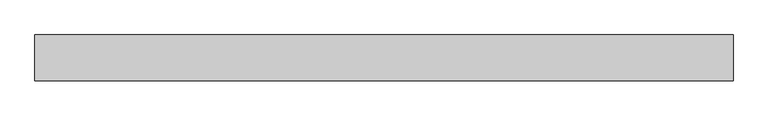
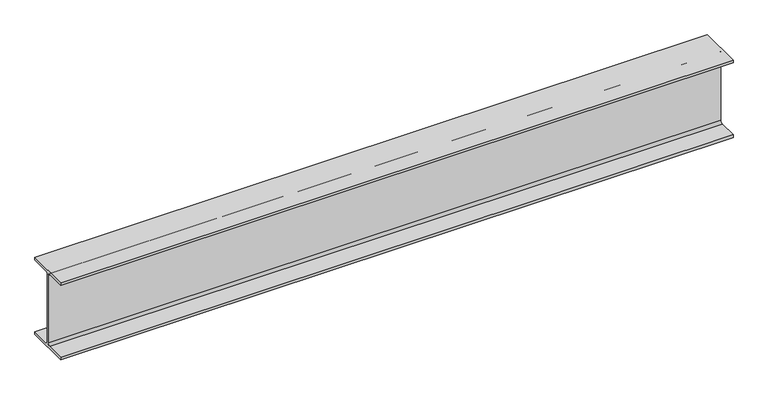
"""IFC4 building model written with IfcOpenShell, lengths in millimetres: beam geometry, Old_Steel Beam_H-KSD3502 : H_SB_ASB_H-200×200x8x12."""

from ifc_helpers import new_model, si_unit, point, frame, frame_2d, origin, place, context, project, spatial, polyline, circle_curve, trimmed, segment, composite_curve, outline, extrude, source, transform, mapped, element, save


def beam_1490ead7(model_context):
    return source(origin(), model_context, "Body", "SweptSolid", [
        extrude(outline(composite_curve([segment(polyline([(82.5, -141.5), (82.5, -151.7), (-82.5, -151.7), (-82.5, -141.5), (-11.9, -141.5)]), True, "CONTINUOUS"), segment(trimmed(circle_curve(frame_2d((-11.9, -132.6)), 8.9), [point((-11.9, -141.5))], [point((-3.0, -132.6))], True, "CARTESIAN"), True, "CONTINUOUS"), segment(polyline([(-3.0, -132.6), (-3.0, 132.6)]), True, "CONTINUOUS"), segment(trimmed(circle_curve(frame_2d((-11.9, 132.6)), 8.9), [point((-3.0, 132.6))], [point((-11.9, 141.5))], True, "CARTESIAN"), True, "CONTINUOUS"), segment(polyline([(-11.9, 141.5), (-82.5, 141.5), (-82.5, 151.7), (82.5, 151.7), (82.5, 141.5), (11.9, 141.5)]), True, "CONTINUOUS"), segment(trimmed(circle_curve(frame_2d((11.9, 132.6)), 8.9), [point((11.9, 141.5))], [point((3.0, 132.6))], True, "CARTESIAN"), True, "CONTINUOUS"), segment(polyline([(3.0, 132.6), (3.0, -132.6)]), True, "CONTINUOUS"), segment(trimmed(circle_curve(frame_2d((11.9, -132.6)), 8.9), [point((3.0, -132.6))], [point((11.9, -141.5))], True, "CARTESIAN"), True, "CONTINUOUS"), segment(polyline([(11.9, -141.5), (82.5, -141.5)]), True, "CONTINUOUS")], self_intersect=False)), frame((-1276.0000495, 0.0, 0.0), z_axis=(1.0, 0.0, 0.0), x_axis=(0.0, 1.0, 0.0)), (0.0, 0.0, 1.0), 2501.5236841),
    ])


if __name__ == "__main__":
    model = new_model("IFC4")
    model_context = context("Model", 3, world=origin())
    ifc_project = project(units=[si_unit("LENGTHUNIT", "METRE", prefix="MILLI")], contexts=[model_context])
    site = spatial("IfcSite", under=ifc_project)
    building = spatial("IfcBuilding", under=site)
    placement = place(None, origin())
    beam_shape = beam_1490ead7(model_context)
    element("IfcBeam", 1, ObjectType="Old_Steel Beam_H-KSD3502 : H_SB_ASB_H-200×200x8x12", at=placement, inside=building, context=model_context, shape_type="MappedRepresentation", body=[
        mapped(beam_shape, transform((0.0, 0.0, 0.0), x_axis=(1.0, 0.0, 0.0), y_axis=(0.0, 1.0, 0.0), z_axis=(0.0, 0.0, 1.0))),
    ])
    save(model, "model.ifc")

# Revit data of these elements
# Type "Old_Steel Beam_H-KSD3502 : H_SB_ASB_H-200×200x8x12"
#   Width = 20.0 cm
#   Web Thickness = 0.8 cm
#   Web Fillet = 1.3 cm
#   Warping Constant = 141376.0 cm⁶
#   Torsional Moment of Inertia = 26.2485 cm⁴
#   Torsional Modulus = 1.0 cm³
#   Section Area = 63.53 cm²
#   Plastic Modulus weak axis = 244.0 cm³
#   Plastic Modulus strong axis = 525.0 cm³
#   Perimeter = 1.16 m²/m
#   Nominal Weight = 49.90 kgf/m
#   Moment of Inertia weak axis = 1600.00 cm⁴
#   Moment of Inertia strong axis = 4720.00 cm⁴
#   Height = 20.0 cm
#   Flange Thickness = 1.2 cm
#   Elastic Modulus weak axis = 160.0 cm³
#   Elastic Modulus strong axis = 472.0 cm³
#   Centroid Vertical = 10.0 cm
#   Centroid Horizontal = 10.0 cm
#   Length [instance default] = 1.5240 m
#   Structural Material [instance default] = Steel, 45-345
#   Assembly Code = ""
# Element 1 (IfcBeam, "Old_Steel Beam_H-KSD3502 : H_SB_ASB_H-200×200x8x12")
#   Structural Material = none
# Materials
#   "Steel, 45-345": class "Metal", colour RGB 189 187 185, transparency 0, Description = "Steel 345 MPa", Cost = 0
